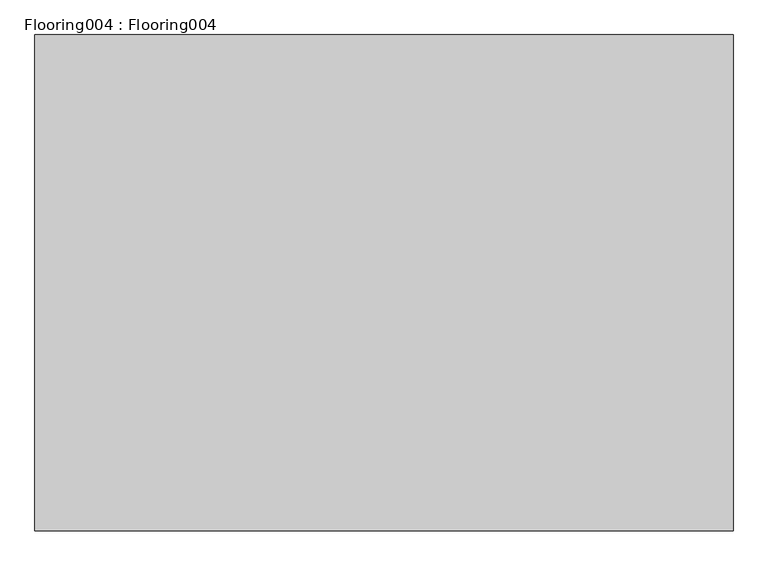
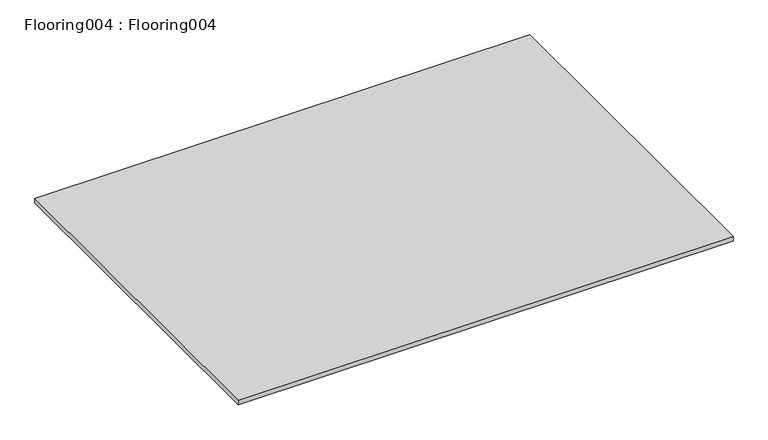
"""IFC4 building model written with IfcOpenShell, lengths in millimetres: proxy geometry, Flooring004 : Flooring004."""

from ifc_helpers import new_model, si_unit, frame, origin, place, context, project, spatial, polyline, outline, extrude, source, transform, mapped, element, save


def flooring004_flooring004_d31bb230(model_context):
    return source(origin(), model_context, "Body", "SweptSolid", [
        extrude(outline(polyline([(12382.7678845, -4250.1925368), (12382.7678845, -2827.7925368), (14383.0178845, -2827.7925368), (14383.0178845, -4250.1925368), (12382.7678845, -4250.1925368)])), frame((0.0, 0.0, 40131.746), z_axis=(0.0, 0.0, 1.0), x_axis=(1.0, 0.0, 0.0)), (0.0, 0.0, 1.0), 19.05),
    ])


if __name__ == "__main__":
    model = new_model("IFC4")
    model_context = context("Model", 3, world=origin())
    ifc_project = project(units=[si_unit("LENGTHUNIT", "METRE", prefix="MILLI")], contexts=[model_context])
    site = spatial("IfcSite", under=ifc_project)
    building = spatial("IfcBuilding", under=site)
    placement = place(None, origin())
    flooring004_flooring004_shape = flooring004_flooring004_d31bb230(model_context)
    element("IfcBuildingElementProxy", 1, Name="Flooring004 : Flooring004", ObjectType="Flooring004 : Flooring004", at=placement, inside=building, context=model_context, shape_type="MappedRepresentation", body=[
        mapped(flooring004_flooring004_shape, transform((0.0, 0.0, 0.0), x_axis=(1.0, 0.0, 0.0), y_axis=(0.0, 1.0, 0.0), z_axis=(0.0, 0.0, 1.0))),
    ])
    save(model, "model.ifc")

# Revit data of these elements
# Type "Flooring004 : Flooring004"
#   NameOverride = "Flooring004"
# Element 1 (IfcBuildingElementProxy, "Flooring004 : Flooring004")
#   Materials on its faces: "WOOD FLOORING (SPEC TBD)"
# Materials
#   "WOOD FLOORING (SPEC TBD)": class "Unassigned", colour RGB 201 162 125, transparency 0
